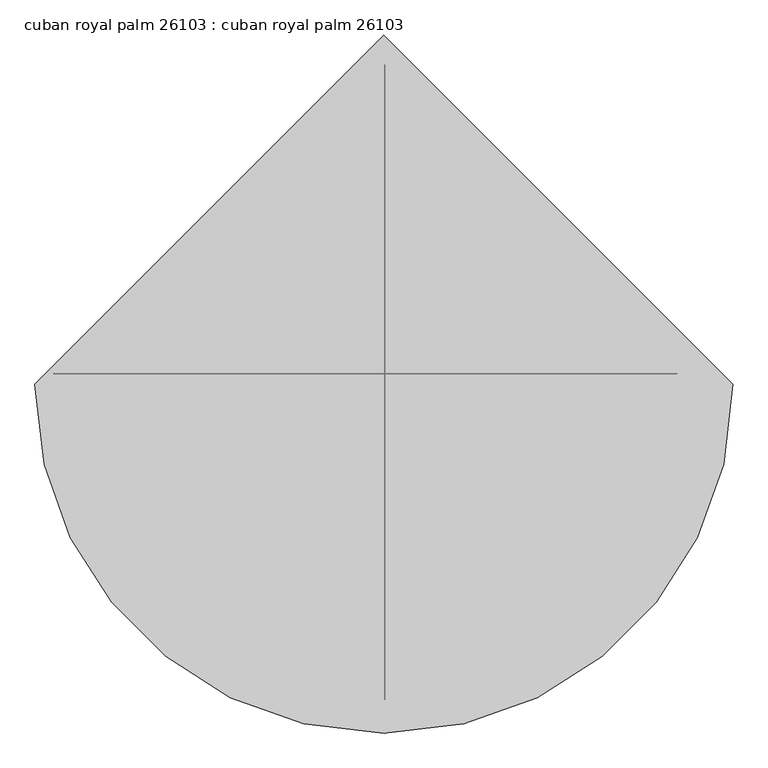
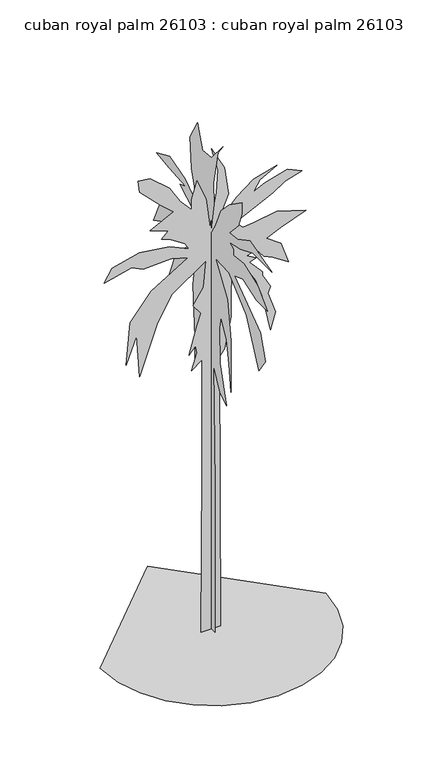
"""IFC4 building model written with IfcOpenShell, lengths in millimetres: proxy geometry, cuban royal palm 26103 : cuban royal palm 26103."""

import ifcopenshell
import ifcopenshell.guid

model = None  # the IFC model being written
_history = None  # IfcOwnerHistory: only IFC2X3 demands one
_inside = {}  # id of a spatial element -> (the spatial element, [elements in it])
_under = {}  # id of a project, library or spatial element -> (it, [spatial elements below it])
_declared = {}  # id of a project -> (the project, [libraries it declares])
_typed = {}  # id of a type object -> (the type object, [elements of that type])
_made_of = {}  # id of a material, layer set ... -> (it, [elements and type objects made of it])


def new_model(schema):
    """Start an empty IFC model of exactly this schema.

    Asked for "IFC4X3", IfcOpenShell would pick the latest addendum, in which some entities
    have other attributes; the version numbers below select the first issue.
    IFC2X3 requires an IfcOwnerHistory on every rooted entity: one is made here for all.
    """
    global model, _history
    if schema == "IFC4X3":
        model = ifcopenshell.file(schema_version=(4, 3, 0, 0))
    else:
        model = ifcopenshell.file(schema=schema)
    _inside.clear()
    _under.clear()
    _declared.clear()
    _typed.clear()
    _made_of.clear()
    _history = None
    if model.schema == "IFC2X3":
        org = make("IfcOrganization", Name="unknown")
        user = make(
            "IfcPersonAndOrganization",
            ThePerson=make("IfcPerson", FamilyName="unknown"),
            TheOrganization=org,
        )
        app = make(
            "IfcApplication",
            ApplicationDeveloper=org,
            Version="unknown",
            ApplicationFullName="unknown",
            ApplicationIdentifier="unknown",
        )
        _history = make(
            "IfcOwnerHistory",
            OwningUser=user,
            OwningApplication=app,
            ChangeAction="ADDED",
            CreationDate=0,
        )
    return model


def make(cls, **values):
    """One entity of the class cls with the attributes given. An attribute that is None is left unset."""
    return model.create_entity(
        cls, **{name: value for name, value in values.items() if value is not None}
    )


def rooted(cls, **values):
    """An entity with a GlobalId (a new one), such as an element, a storey or a relation."""
    return make(cls, GlobalId=ifcopenshell.guid.new(), OwnerHistory=_history, **values)


def si_unit(unit_type, name, prefix=None):
    """IfcSIUnit, for example si_unit("LENGTHUNIT", "METRE", prefix="MILLI")."""
    return make("IfcSIUnit", UnitType=unit_type, Prefix=prefix, Name=name)


def assignment(units):
    """IfcUnitAssignment: the units of a project."""
    return None if units is None else make("IfcUnitAssignment", Units=units)


def point(xyz):
    """IfcCartesianPoint."""
    return None if xyz is None else make("IfcCartesianPoint", Coordinates=xyz)


def direction(xyz):
    """IfcDirection."""
    return None if xyz is None else make("IfcDirection", DirectionRatios=xyz)


def frame(location, z_axis=None, x_axis=None):
    """IfcAxis2Placement3D, a coordinate frame: its origin and axes. An axis left out is left unset."""
    return make(
        "IfcAxis2Placement3D",
        Location=point(location),
        Axis=direction(z_axis),
        RefDirection=direction(x_axis),
    )


def origin():
    """The frame at (0, 0, 0) with its axes left unset."""
    return frame((0.0, 0.0, 0.0))


def place(relative_to, where):
    """IfcLocalPlacement: puts the frame where relative to a parent placement (None: the world)."""
    return make(
        "IfcLocalPlacement", PlacementRelTo=relative_to, RelativePlacement=where
    )


def context(
    kind, dimensions, precision=None, world=None, true_north=None, identifier=None
):
    """IfcGeometricRepresentationContext, for example the 3D "Model" context."""
    return make(
        "IfcGeometricRepresentationContext",
        ContextIdentifier=identifier,
        ContextType=kind,
        CoordinateSpaceDimension=dimensions,
        Precision=precision,
        WorldCoordinateSystem=world,
        TrueNorth=true_north,
    )


def project(units=None, contexts=None):
    """IfcProject with its units and contexts."""
    return rooted(
        "IfcProject",
        Name="project",
        RepresentationContexts=contexts,
        UnitsInContext=assignment(units),
    )


def spatial(cls, under=None, at=None, **own):
    """A site, building, storey or space (cls), placed at a placement, below another one or the project."""
    s = rooted(cls, ObjectPlacement=at, **own)
    if under is not None:
        _under.setdefault(under.id(), (under, []))[1].append(s)
    return s


def point_list(points):
    """IfcCartesianPointList2D or 3D."""
    cls = (
        "IfcCartesianPointList2D" if len(points[0]) == 2 else "IfcCartesianPointList3D"
    )
    return make(cls, CoordList=points)


def triangles(points, corners, closed=None, point_numbers=None):
    """IfcTriangulatedFaceSet: each triangle names its three corners, points numbered from 1."""
    return make(
        "IfcTriangulatedFaceSet",
        Coordinates=point_list(points),
        Closed=closed,
        CoordIndex=corners,
        PnIndex=point_numbers,
    )


def shape(context_of_items, identifier, shape_type, items):
    """IfcShapeRepresentation: the items that make up one representation, for example the "Body"."""
    return make(
        "IfcShapeRepresentation",
        ContextOfItems=context_of_items,
        RepresentationIdentifier=identifier,
        RepresentationType=shape_type,
        Items=items,
    )


def source(mapping_origin, context_of_items, identifier, shape_type, items):
    """IfcRepresentationMap: a shape defined once, which mapped items show again and again."""
    return make(
        "IfcRepresentationMap",
        MappingOrigin=mapping_origin,
        MappedRepresentation=shape(context_of_items, identifier, shape_type, items),
    )


def transform(
    local_origin,
    x_axis=None,
    y_axis=None,
    z_axis=None,
    scale=None,
    scale2=None,
    scale3=None,
    uniform=True,
):
    """IfcCartesianTransformationOperator3D, or its non-uniform kind. x_axis, y_axis, z_axis: its Axis1, 2, 3."""
    if uniform:
        return make(
            "IfcCartesianTransformationOperator3D",
            Axis1=direction(x_axis),
            Axis2=direction(y_axis),
            LocalOrigin=point(local_origin),
            Scale=scale,
            Axis3=direction(z_axis),
        )
    return make(
        "IfcCartesianTransformationOperator3DnonUniform",
        Axis1=direction(x_axis),
        Axis2=direction(y_axis),
        LocalOrigin=point(local_origin),
        Scale=scale,
        Axis3=direction(z_axis),
        Scale2=scale2,
        Scale3=scale3,
    )


def mapped(mapping_source, mapping_target):
    """IfcMappedItem: shows the shape of a source again, moved by a transform."""
    return make(
        "IfcMappedItem", MappingSource=mapping_source, MappingTarget=mapping_target
    )


def made_of(thing, what):
    """Note that an element or type object is made of a material, layer set ...; save() writes the relation."""
    if what is not None:
        _made_of.setdefault(what.id(), (what, []))[1].append(thing)
    return thing


def element(
    cls,
    number,
    at=None,
    inside=None,
    cuts=None,
    type_object=None,
    material=None,
    context=None,
    identifier="Body",
    shape_type=None,
    held_by="IfcProductDefinitionShape",
    body=None,
    shapes=None,
    **own,
):
    """One element of the class cls, such as IfcWall. Its Tag is "e" and its number.

    at: its placement. inside: the storey or other place that contains it. cuts: it is an
    opening in that element (IfcRelVoidsElement). A single representation is given by context,
    identifier, shape_type and body (its items); several are given by shapes. held_by: the class
    of the entity that holds the representations. save() writes the other relations.
    """
    e = rooted(cls, Tag="e%d" % number, ObjectPlacement=at, **own)
    if body is not None:
        shapes = [shape(context, identifier, shape_type, body)]
    if shapes is not None:
        e.Representation = make(held_by, Representations=shapes)
    if inside is not None:
        _inside.setdefault(inside.id(), (inside, []))[1].append(e)
    if cuts is not None:
        rooted(
            "IfcRelVoidsElement", RelatingBuildingElement=cuts, RelatedOpeningElement=e
        )
    if type_object is not None:
        _typed.setdefault(type_object.id(), (type_object, []))[1].append(e)
    return made_of(e, material)


def aggregate(whole, parts):
    """IfcRelAggregates: a whole, such as a stair, and the parts it consists of."""
    return rooted("IfcRelAggregates", RelatingObject=whole, RelatedObjects=parts)


def save(model, path):
    """Write the relations noted so far, then the file.

    IfcRelAggregates (storeys below a building ...), IfcRelContainedInSpatialStructure (elements
    in a storey), IfcRelDefinesByType, IfcRelAssociatesMaterial and IfcRelDeclares: one each for
    every whole, place, type object, material and project.
    """
    for whole, parts in _under.values():
        aggregate(whole, parts)
    for where, things in _inside.values():
        rooted(
            "IfcRelContainedInSpatialStructure",
            RelatedElements=things,
            RelatingStructure=where,
        )
    for kind, things in _typed.values():
        rooted("IfcRelDefinesByType", RelatedObjects=things, RelatingType=kind)
    for what, things in _made_of.values():
        rooted("IfcRelAssociatesMaterial", RelatedObjects=things, RelatingMaterial=what)
    for by, libraries in _declared.values():
        rooted("IfcRelDeclares", RelatingContext=by, RelatedDefinitions=libraries)
    model.write(path)


def cuban_royal_palm_26103_cuban_royal_palm_26103_6f0ceb55(model_context):
    return source(origin(), model_context, "Body", "Tessellation", [
        triangles([(-54.3826135, -0.017491, 0.0009437), (-150.0419681, -0.0174994, 0.0009479), (-130.9099418, -0.0179382, 2494.6483109), (-130.9096875, -0.0182426, 4197.3711227), (-283.9640988, -0.0182154, 4082.5885941), (-207.4377743, -0.0182632, 4331.3053894), (-226.5690375, -0.0182829, 4446.0876274), (-322.2291687, -0.0182582, 4331.3053894), (-207.4375199, -0.0183385, 4752.2081863), (-150.0417137, -0.0183718, 4924.3947693), (-264.8328356, -0.0183942, 5077.4551941), (-111.778179, -0.0184419, 5307.0196701), (-73.5143854, -0.0185154, 5708.7968903), (-570.9431663, -0.0184321, 5364.4237244), (-781.3921303, -0.0183579, 5000.9249817), (-1049.2399527, -0.0182128, 4254.775177), (-1087.5024427, -0.0183274, 4905.2686111), (-1240.5575626, -0.0182489, 4503.4916817), (-1183.1638275, -0.0183643, 5134.8336685), (-877.0535151, -0.0184461, 5517.4841492), (-341.3604137, -0.0185277, 5842.7305756), (-590.0744476, -0.0185305, 5919.260788), (-991.8436014, -0.0185095, 5900.10905), (-1164.030039, -0.0185156, 5976.6392624), (-1565.7991928, -0.018481, 5880.9828918), (-1451.0091064, -0.0185202, 6072.2956329), (-1049.2399527, -0.0185549, 6167.9775833), (-609.2056927, -0.0185639, 6110.5735291), (-322.2291687, -0.0185524, 5976.6392624), (-379.6254836, -0.018567, 6072.2956329), (-609.2056927, -0.0185844, 6225.3560577), (-723.9983225, -0.0185862, 6263.6339539), (-628.3394812, -0.0186075, 6359.2903244), (-896.1847601, -0.0186129, 6454.9461136), (-551.8119212, -0.0186587, 6627.1326965), (-743.1295675, -0.0186811, 6799.3192795), (-1049.2399527, -0.0187225, 7105.4395477), (-1068.3711977, -0.0187524, 7277.6261307), (-896.1847601, -0.0187566, 7258.4743927), (-609.2056927, -0.0187246, 7009.7581787), (-456.1505364, -0.0186868, 6761.0413834), (-283.9640988, -0.0186602, 6569.7286423), (-283.9640988, -0.0186875, 6722.7890671), (-207.4375199, -0.0187388, 6990.6320206), (-73.5143854, -0.0186865, 6665.3850128), (-16.1188494, -0.0186069, 6206.2298996), (79.5405301, -0.0187, 6703.6629089), (98.6725473, -0.0187624, 7048.0354935), (3.0131737, -0.0188232, 7411.5348175), (194.3319064, -0.0187666, 7048.0354935), (251.7277126, -0.0186938, 6627.1326965), (79.5405301, -0.018611, 6206.2298996), (366.5190888, -0.0186818, 6531.476326), (615.2330864, -0.0187268, 6722.7890671), (959.6059616, -0.018759, 6818.4454376), (710.8919277, -0.0187242, 6684.5367508), (615.2330864, -0.0186926, 6531.476326), (787.419524, -0.0187138, 6608.0065384), (1112.6611542, -0.0187452, 6703.6629089), (1323.1125526, -0.0187373, 6608.0065384), (1074.3985914, -0.0187127, 6531.476326), (902.2121538, -0.0186847, 6416.6687988), (347.3878438, -0.0186125, 6148.8258453), (462.1779302, -0.018597, 6034.0433167), (615.2330864, -0.0186071, 6053.1694748), (959.6059616, -0.0186324, 6110.5735291), (1380.5089039, -0.0186269, 5976.6392624), (1017.0023129, -0.018587, 5842.7305756), (806.550769, -0.0185607, 5747.074205), (1017.0023129, -0.0185426, 5594.0143616), (1131.7923992, -0.0184894, 5268.7673538), (902.2121538, -0.0185068, 5421.8277786), (768.288279, -0.0185112, 5479.2062531), (615.2330864, -0.0185387, 5670.544574), (615.2330864, -0.0185284, 5613.1405197), (519.5742451, -0.0185174, 5574.8882034), (653.4956491, -0.0185096, 5498.357991), (557.8367715, -0.0184985, 5460.0800949), (749.1570339, -0.0184693, 5249.6411957), (749.1570339, -0.018459, 5192.2371414), (863.9471203, -0.0184264, 4981.7988235), (825.6846302, -0.0184076, 4886.142453), (940.4747166, -0.0183545, 4560.8957359), (863.9471203, -0.0183067, 4312.1792313), (749.1570339, -0.0184009, 4866.990715), (653.4956491, -0.018448, 5153.9848251), (481.3092115, -0.0184918, 5440.9539368), (309.1227739, -0.0184979, 5517.4841492), (289.9915107, -0.0184287, 5134.8336685), (289.9915107, -0.0183534, 4713.9558701), (194.3319064, -0.0182671, 4254.775177), (117.8043192, -0.0182467, 4159.1188065), (136.9360911, -0.0175052, 0.0009354), (-0.003708, 89.5986644, 0.000495), (-0.0037084, 163.6334895, 0.0005082), (-0.003708, 163.6334895, 1826.7789024), (-0.003706, 145.1250443, 4288.4300995), (-0.0037076, 219.1593699, 4177.3813545), (-0.0037057, 404.2456741, 3788.6856033), (-0.0037071, 404.2456741, 4251.4224747), (-0.0037068, 459.7725537, 5028.7883972), (-0.0037083, 385.7367022, 5565.5410995), (-0.0037091, 533.8058619, 5398.9425476), (-0.0037068, 792.9287807, 4862.190136), (-0.0037064, 1089.0671001, 4492.0362762), (-0.0037084, 1311.1695316, 4140.3737297), (-0.0037071, 1052.0491562, 4843.6988228), (-0.0037074, 885.4710245, 5250.8858871), (-0.0037074, 515.2968899, 5621.065036), (-0.003709, 681.8750216, 5584.0318314), (-0.0037073, 903.9799965, 5565.5410995), (-0.0037076, 1107.5760721, 5602.5487244), (-0.0037076, 1459.2413074, 5417.4588593), (-0.0037087, 1274.1542038, 5824.6462143), (-0.0037067, 1070.5581282, 5824.6462143), (-0.0037071, 996.5223129, 6139.3008453), (-0.0037076, 644.859621, 6065.2600159), (-0.0037089, 422.7546461, 6176.3084702), (-0.0037091, 792.9287807, 6379.9146469), (-0.0037059, 644.859621, 6435.4391647), (-0.0037081, 1052.0491562, 6472.4467896), (-0.0037064, 1385.2054195, 6509.4799942), (-0.0037073, 1052.0491562, 6657.5366547), (-0.0037075, 663.368593, 6546.487619), (-0.0037092, 348.7187945, 6324.3907104), (-0.003707, 496.7904977, 6805.6183136), (-0.0037068, 533.8058619, 7268.3296051), (-0.0037076, 348.7187945, 7601.4755493), (-0.0037068, 311.703394, 7490.427095), (-0.0037069, 219.1593699, 7249.8132935), (-0.0037086, -2.9445681, 7268.3296051), (-0.0037062, -299.0821622, 7619.9924423), (-0.0037078, -169.5227376, 7453.4194702), (-0.0037084, -58.4704863, 6916.6673492), (-0.0037085, -76.9791948, 6602.0121368), (-0.003709, 15.5640629, 6083.7763275), (-0.0037058, -113.9968663, 6287.3575058), (-0.0037085, -243.5573174, 6602.0121368), (-0.0037085, -465.6602757, 6824.1096268), (-0.003709, -780.3075308, 7046.2321152), (-0.003709, -780.3075308, 6879.6341446), (-0.0037083, -687.765287, 6639.0453415), (-0.0037091, -465.6602757, 6398.4315399), (-0.0037063, -669.256315, 6416.9228531), (-0.0037092, -983.9036064, 6583.4958252), (-0.0037074, -1539.164772, 6435.4391647), (-0.0037081, -1057.9394217, 6435.4391647), (-0.0037072, -743.2921303, 6305.8738174), (-0.0037083, -465.6602757, 6250.3492996), (-0.0037076, -558.2050993, 6194.8253632), (-0.003708, -558.2050993, 6102.2932205), (-0.0037077, -835.8344467, 6139.3008453), (-0.0037071, -1187.4996094, 6009.735498), (-0.0037064, -1428.1110855, 5769.1216965), (-0.0037087, -1150.4816654, 5769.1216965), (-0.0037066, -798.8165028, 5880.1701508), (-0.0037081, -595.2230069, 5806.1549011), (-0.0037069, -1243.0264526, 5324.9267166), (-0.0037071, -1372.586713, 4954.7475677), (-0.0037067, -1206.0085814, 4714.1337662), (-0.0037072, -891.36129, 5380.4512344), (-0.0037069, -447.1538472, 5769.1216965), (-0.003706, -113.9968663, 5787.6380081), (-0.0037066, -410.1359396, 5324.9267166), (-0.0037068, -502.6781834, 4751.141391), (-0.0037091, -502.6781834, 3955.2841553), (-0.0037069, -447.1538472, 4362.470929), (-0.003708, -391.6269676, 4695.6171638), (-0.0037083, -243.5573174, 4954.7475677), (-0.0037075, -206.5399003, 4769.6579933), (-0.0037065, -225.0485998, 4232.9058723), (-0.0037092, -391.6269676, 3677.6368584), (-0.0037079, -225.0485998, 3788.6856033), (-0.0037085, -58.4704863, 4103.3405251), (-0.0037063, -95.4881577, 2289.4952808), (-0.0037089, -95.4881577, 0.0004619), (-1653.0963352, -49.1291369, 0.0005424), (-1609.512513, -426.8745255, 0.000473), (-1485.3879673, -773.7746447, 0.0004055), (-1290.6616264, -1079.890044, 0.0003423), (-1035.2724913, -1335.2792519, 0.0002854), (-729.1570919, -1530.0055927, 0.0002372), (-382.2594435, -1654.1301384, 0.0001999), (-4.5121786, -1697.7139606, 0.0001756), (373.234849, -1654.1301384, 0.0001668), (720.1324247, -1530.0055927, 0.0001739), (1026.2478968, -1335.2792519, 0.0001953), (1281.6370319, -1079.890044, 0.0002298), (1476.3633728, -773.7746447, 0.000276), (1600.4879185, -426.8745255, 0.0003326), (1644.0717407, -49.1291369, 0.0003983), (-4.5124832, 1599.4541153, 0.0003027)], [[54, 55, 56], [48, 49, 50], [17, 18, 19], [15, 16, 17], [7, 8, 9], [83, 84, 85], [82, 83, 85], [4, 5, 6], [70, 71, 72], [66, 67, 68], [43, 44, 45], [59, 60, 61], [24, 25, 26], [24, 26, 27], [33, 34, 35], [76, 77, 78], [58, 59, 61], [58, 61, 62], [31, 32, 33], [42, 43, 45], [42, 45, 46], [37, 38, 39], [54, 56, 57], [53, 54, 57], [23, 24, 27], [23, 27, 28], [22, 23, 28], [22, 28, 29], [21, 22, 29], [58, 62, 63], [57, 58, 63], [53, 57, 63], [52, 53, 63], [36, 37, 39], [36, 39, 40], [36, 40, 41], [35, 36, 41], [35, 41, 42], [69, 70, 72], [69, 72, 73], [69, 73, 74], [65, 66, 68], [65, 68, 69], [65, 69, 74], [64, 65, 74], [47, 48, 50], [47, 50, 51], [46, 47, 51], [46, 51, 52], [33, 35, 42], [82, 85, 86], [81, 82, 86], [80, 81, 86], [33, 42, 46], [31, 33, 46], [30, 31, 46], [29, 30, 46], [15, 17, 19], [15, 19, 20], [14, 15, 20], [14, 20, 21], [13, 14, 21], [92, 93, 1], [92, 1, 2], [92, 2, 3], [92, 3, 4], [80, 86, 87], [79, 80, 87], [78, 79, 87], [76, 78, 87], [76, 87, 88], [13, 21, 29], [13, 29, 46], [13, 46, 52], [13, 52, 63], [13, 63, 64], [13, 64, 74], [13, 74, 75], [13, 75, 76], [13, 76, 88], [12, 13, 88], [12, 88, 89], [11, 12, 89], [10, 11, 89], [10, 89, 90], [9, 10, 90], [9, 90, 91], [7, 9, 91], [6, 7, 91], [4, 6, 91], [92, 4, 91], [131, 132, 133], [165, 166, 167], [105, 106, 107], [145, 146, 147], [165, 167, 168], [98, 99, 100], [131, 133, 134], [121, 122, 123], [104, 105, 107], [112, 113, 114], [171, 172, 173], [171, 173, 174], [153, 154, 155], [127, 128, 129], [118, 119, 120], [112, 114, 115], [139, 140, 141], [139, 141, 142], [159, 160, 161], [158, 159, 161], [157, 158, 161], [157, 161, 162], [104, 107, 108], [103, 104, 108], [103, 108, 109], [102, 103, 109], [127, 129, 130], [121, 123, 124], [120, 121, 124], [120, 124, 125], [118, 120, 125], [153, 155, 156], [152, 153, 156], [151, 152, 156], [151, 156, 157], [126, 127, 130], [145, 147, 148], [144, 145, 148], [144, 148, 149], [143, 144, 149], [139, 142, 143], [138, 139, 143], [137, 138, 143], [137, 143, 149], [175, 176, 94], [175, 94, 95], [175, 95, 96], [175, 96, 97], [174, 175, 97], [111, 112, 115], [115, 116, 117], [111, 115, 117], [110, 111, 117], [109, 110, 117], [165, 168, 169], [164, 165, 169], [130, 131, 134], [126, 130, 134], [126, 134, 135], [125, 126, 135], [125, 135, 136], [118, 125, 136], [151, 157, 162], [171, 174, 97], [170, 171, 97], [109, 117, 118], [109, 118, 136], [102, 109, 136], [97, 98, 100], [97, 100, 101], [170, 97, 101], [169, 170, 101], [169, 101, 102], [164, 169, 102], [163, 164, 102], [163, 102, 136], [151, 162, 163], [151, 163, 136], [151, 136, 137], [151, 137, 149], [151, 149, 150], [191, 192, 177], [190, 191, 177], [190, 177, 178], [189, 190, 178], [189, 178, 179], [189, 179, 180], [188, 189, 180], [187, 188, 180], [187, 180, 181], [187, 181, 182], [187, 182, 183], [187, 183, 184], [187, 184, 185], [187, 185, 186]], closed=False),
    ])


if __name__ == "__main__":
    model = new_model("IFC4")
    model_context = context("Model", 3, world=origin())
    ifc_project = project(units=[si_unit("LENGTHUNIT", "METRE", prefix="MILLI")], contexts=[model_context])
    site = spatial("IfcSite", under=ifc_project)
    building = spatial("IfcBuilding", under=site)
    placement = place(None, origin())
    cuban_royal_palm_26103_cuban_royal_palm_26103_shape = cuban_royal_palm_26103_cuban_royal_palm_26103_6f0ceb55(model_context)
    element("IfcBuildingElementProxy", 1, Name="cuban royal palm 26103 : cuban royal palm 26103", ObjectType="cuban royal palm 26103 : cuban royal palm 26103", at=placement, inside=building, context=model_context, shape_type="MappedRepresentation", body=[
        mapped(cuban_royal_palm_26103_cuban_royal_palm_26103_shape, transform((0.0, 0.0, 0.0), x_axis=(1.0, 0.0, 0.0), y_axis=(0.0, 1.0, 0.0), z_axis=(0.0, 0.0, 1.0))),
    ])
    save(model, "model.ifc")

# Revit data of these elements
# Type "cuban royal palm 26103 : cuban royal palm 26103"
#   built-in parameter 1005195 = "RPC-16-FVGV-NKG0-7NHH-C000-ST1L-LVER-AU"
#   Height = 0
